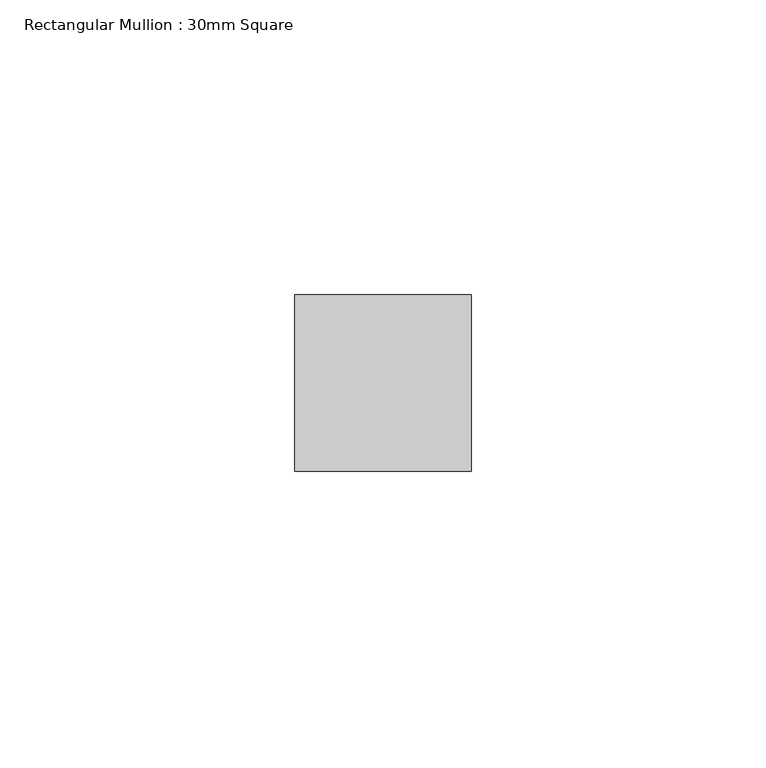
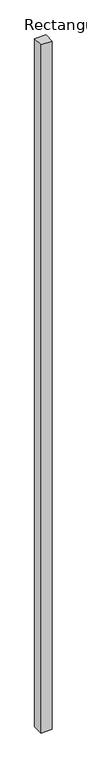
"""IFC4 building model written with IfcOpenShell, lengths in millimetres: member geometry, Rectangular Mullion : 30mm Square."""

from ifc_helpers import new_model, si_unit, frame, origin, place, context, project, spatial, polyline, outline, extrude, source, transform, mapped, element, save


def rectangular_mullion_30mm_square_fd0918f0(model_context):
    return source(origin(), model_context, "Body", "SweptSolid", [
        extrude(outline(polyline([(15.0, 15.0), (15.0, -15.0), (-15.0, -15.0), (-15.0, 15.0), (15.0, 15.0)])), frame((0.0, 0.0, -1962.7394135), z_axis=(0.0, 0.0, 1.0), x_axis=(1.0, 0.0, 0.0)), (0.0, 0.0, 1.0), 1962.7394135),
    ])


if __name__ == "__main__":
    model = new_model("IFC4")
    model_context = context("Model", 3, world=origin())
    ifc_project = project(units=[si_unit("LENGTHUNIT", "METRE", prefix="MILLI")], contexts=[model_context])
    site = spatial("IfcSite", under=ifc_project)
    building = spatial("IfcBuilding", under=site)
    placement = place(None, origin())
    rectangular_mullion_30mm_square_shape = rectangular_mullion_30mm_square_fd0918f0(model_context)
    element("IfcMember", 1, ObjectType="Rectangular Mullion : 30mm Square", at=placement, inside=building, context=model_context, shape_type="MappedRepresentation", body=[
        mapped(rectangular_mullion_30mm_square_shape, transform((0.0, 0.0, 0.0), x_axis=(1.0, 0.0, 0.0), y_axis=(0.0, 1.0, 0.0), z_axis=(0.0, 0.0, 1.0))),
    ])
    save(model, "model.ifc")

# Revit data of these elements
# Type "Rectangular Mullion : 30mm Square"
#   built-in parameter 1007304 = 0.0984252 (stored number, unit not read)
#   built-in parameter 1007301 = 0.0492126 (stored number, unit not read)
#   built-in parameter 1007300 = 0.0492126 (stored number, unit not read)
# Element 1 (IfcMember, "Rectangular Mullion : 30mm Square")
#   Materials on its faces: "Aluminum"
# Materials
#   "Aluminum": class "Metal", colour RGB 244 244 244, transparency 0, Description = "Aluminum 6061", Cost = 0
